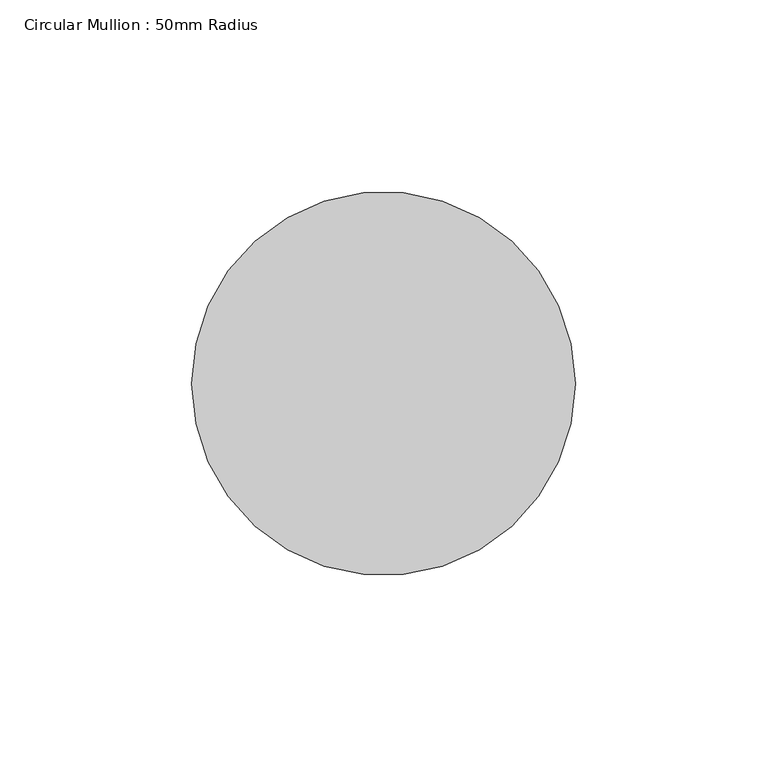
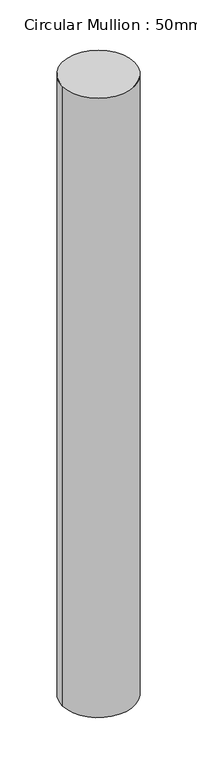
"""IFC4 building model written with IfcOpenShell, lengths in millimetres: member geometry, Circular Mullion : 50mm Radius."""

from ifc_helpers import new_model, si_unit, point, frame, origin, origin_2d, place, context, project, spatial, circle_curve, trimmed, segment, composite_curve, outline, extrude, source, transform, mapped, element, save


def circular_mullion_50mm_radius_6d1b0beb(model_context):
    return source(origin(), model_context, "Body", "SweptSolid", [
        extrude(outline(composite_curve([segment(trimmed(circle_curve(origin_2d(), 50.0), [point((50.0, 0.0))], [point((-50.0, 0.0))], False, "CARTESIAN"), True, "CONTINUOUS"), segment(trimmed(circle_curve(origin_2d(), 50.0), [point((-50.0, 0.0))], [point((50.0, 0.0))], False, "CARTESIAN"), True, "CONTINUOUS")], self_intersect=False)), frame((0.0, 0.0, -907.3629445), z_axis=(0.0, 0.0, 1.0), x_axis=(1.0, 0.0, 0.0)), (0.0, 0.0, 1.0), 907.3629445),
    ])


if __name__ == "__main__":
    model = new_model("IFC4")
    model_context = context("Model", 3, world=origin())
    ifc_project = project(units=[si_unit("LENGTHUNIT", "METRE", prefix="MILLI")], contexts=[model_context])
    site = spatial("IfcSite", under=ifc_project)
    building = spatial("IfcBuilding", under=site)
    placement = place(None, origin())
    circular_mullion_50mm_radius_shape = circular_mullion_50mm_radius_6d1b0beb(model_context)
    element("IfcMember", 1, ObjectType="Circular Mullion : 50mm Radius", at=placement, inside=building, context=model_context, shape_type="MappedRepresentation", body=[
        mapped(circular_mullion_50mm_radius_shape, transform((0.0, 0.0, 0.0), x_axis=(1.0, 0.0, 0.0), y_axis=(0.0, 1.0, 0.0), z_axis=(0.0, 0.0, 1.0))),
    ])
    save(model, "model.ifc")

# Revit data of these elements
# Type "Circular Mullion : 50mm Radius"
#   built-in parameter 1007350 = 0.164042 (stored number, unit not read)
# Element 1 (IfcMember, "Circular Mullion : 50mm Radius")
#   Materials on its faces: "Aluminium"
# Materials
#   "Aluminium": class "Metal", colour RGB 247 247 247, transparency 0, Description = "Aluminium 6061", Cost = 0
